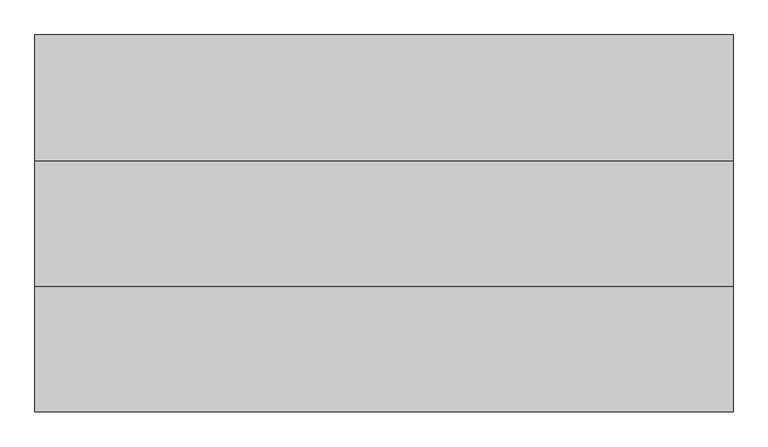
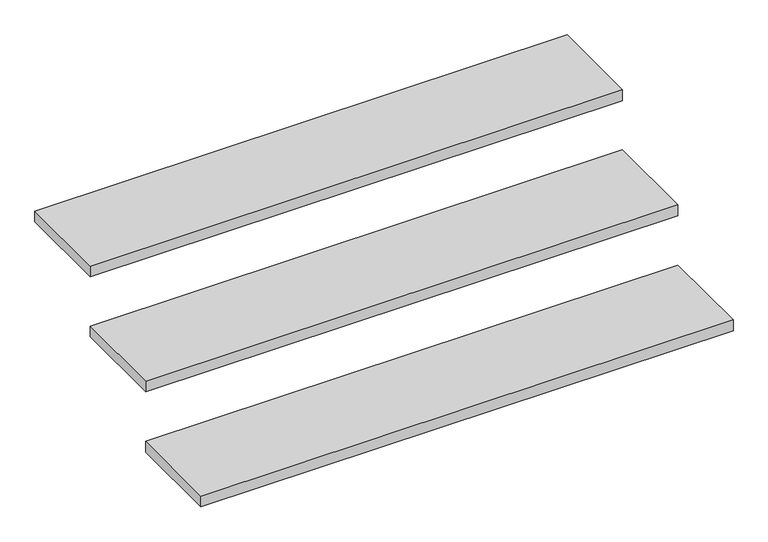
"""IFC4 building model written with IfcOpenShell, lengths in millimetres: stair flight geometry."""

from ifc_helpers import new_model, si_unit, frame, origin, place, context, project, spatial, polyline, outline, extrude, source, transform, mapped, element, save


def stair_flight_10571817(model_context):
    return source(origin(), model_context, "Body", "SweptSolid", [
        extrude(outline(polyline([(17005.3403387, 2217.6066446), (18505.3403387, 2217.6066446), (18505.3403387, 1947.6066446), (17005.3403387, 1947.6066446), (17005.3403387, 2217.6066446)])), frame((0.0, 0.0, 15909.7582418), z_axis=(0.0, 0.0, 1.0), x_axis=(1.0, 0.0, 0.0)), (0.0, 0.0, 1.0), 32.0),
        extrude(outline(polyline([(17005.3403387, 2487.6066446), (18505.3403387, 2487.6066446), (18505.3403387, 2217.6066446), (17005.3403387, 2217.6066446), (17005.3403387, 2487.6066446)])), frame((0.0, 0.0, 16088.8791209), z_axis=(0.0, 0.0, 1.0), x_axis=(1.0, 0.0, 0.0)), (0.0, 0.0, 1.0), 32.0),
        extrude(outline(polyline([(17005.3403387, 2757.6066446), (18505.3403387, 2757.6066446), (18505.3403387, 2487.6066446), (17005.3403387, 2487.6066446), (17005.3403387, 2757.6066446)])), frame((0.0, 0.0, 16268.0), z_axis=(0.0, 0.0, 1.0), x_axis=(1.0, 0.0, 0.0)), (0.0, 0.0, 1.0), 32.0),
    ])


if __name__ == "__main__":
    model = new_model("IFC4")
    model_context = context("Model", 3, world=origin())
    ifc_project = project(units=[si_unit("LENGTHUNIT", "METRE", prefix="MILLI")], contexts=[model_context])
    site = spatial("IfcSite", under=ifc_project)
    building = spatial("IfcBuilding", under=site)
    placement = place(None, origin())
    stair_flight_shape = stair_flight_10571817(model_context)
    element("IfcStairFlight", 1, at=placement, inside=building, context=model_context, shape_type="MappedRepresentation", body=[
        mapped(stair_flight_shape, transform((0.0, 0.0, 0.0), x_axis=(1.0, 0.0, 0.0), y_axis=(0.0, 1.0, 0.0), z_axis=(0.0, 0.0, 1.0))),
    ])
    save(model, "model.ifc")

# Revit data of these elements
# Element 1 (IfcStairFlight)
#   Materials on its faces: "철강"
# Materials
#   "철강": class "Generic", colour RGB 143 142 141, transparency 0, Description = "철골+가공조립+세우기", Cost = 0
